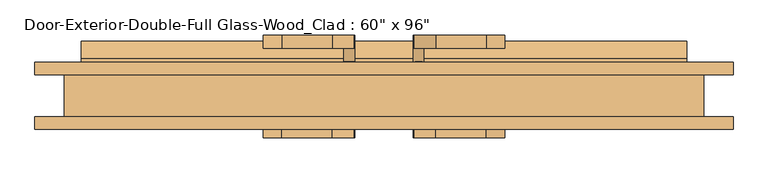
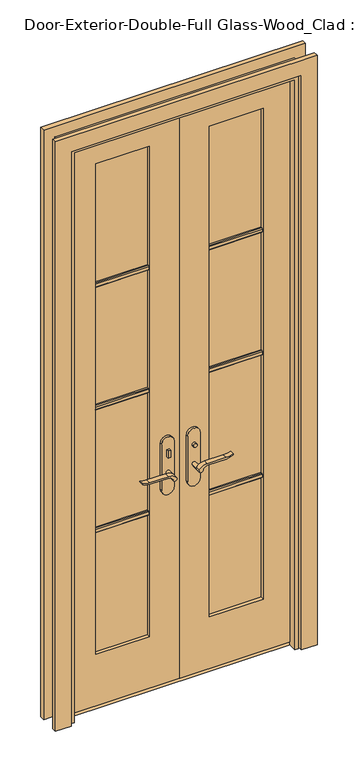
"""IFC4 building model written with IfcOpenShell, lengths in millimetres: door geometry."""

from ifc_helpers import new_model, si_unit, point, frame, frame_2d, origin, place, context, project, spatial, polyline, circle_curve, trimmed, segment, composite_curve, outline, extrude, faceted_brep, source, transform, mapped, element, save


def door_199e0ab3(model_context):
    return source(origin(), model_context, "Body", "SolidModel", [
        extrude(outline(polyline([(19.05, 12.7), (53.975, 12.7), (79.375, 0.0), (-6.35, 0.0), (19.05, 12.7)])), frame((-457.2, 0.0, 0.0), z_axis=(1.0, 0.0, 0.0), x_axis=(0.0, 1.0, 0.0)), (0.0, 0.0, 1.0), 914.4),
        extrude(outline(polyline([(-47.4019111, -26.35), (-57.4019111, -26.35), (-57.4019111, -16.35), (-47.4019111, -16.35), (-47.4019111, -26.35)])), frame((0.0, 0.0, 981.9), z_axis=(0.0, 0.0, 1.0), x_axis=(1.0, 0.0, 0.0)), (0.0, 0.0, 1.0), 30.0),
        extrude(outline(composite_curve([segment(trimmed(circle_curve(frame_2d((996.9, -52.4019111)), 8.0), [point((996.9, -60.4019111))], [point((996.9, -44.4019111))], False, "CARTESIAN"), True, "CONTINUOUS"), segment(trimmed(circle_curve(frame_2d((996.9, -52.4019111)), 8.0), [point((996.9, -44.4019111))], [point((996.9, -60.4019111))], False, "CARTESIAN"), True, "CONTINUOUS")], self_intersect=False)), frame((0.0, 38.575, 0.0), z_axis=(0.0, 1.0, 0.0), x_axis=(0.0, 0.0, 1.0)), (0.0, 0.0, 1.0), 10.0),
        extrude(outline(composite_curve([segment(trimmed(circle_curve(frame_2d((897.1555521, -76.0694241)), 37.2832219), [point((919.0523287, -45.8937749))], [point((934.4, -77.7693445))], False, "CARTESIAN"), True, "CONTINUOUS"), segment(polyline([(934.4, -77.7693445), (934.4, -154.045502)]), True, "CONTINUOUS"), segment(trimmed(circle_curve(frame_2d((1017.6850638, -153.9791202)), 83.2850902), [point((934.4, -154.045502))], [point((939.4, -182.4019111))], True, "CARTESIAN"), True, "CONTINUOUS"), segment(polyline([(939.4, -182.4019111), (936.6135558, -182.4019111)]), True, "CONTINUOUS"), segment(trimmed(circle_curve(frame_2d((986.6709207, -150.4622499)), 59.3791355), [point((936.6135558, -182.4019111))], [point((927.4, -154.045502))], False, "CARTESIAN"), True, "CONTINUOUS"), segment(polyline([(927.4, -154.045502), (927.4, -77.7881013)]), True, "CONTINUOUS"), segment(trimmed(circle_curve(frame_2d((909.2738613, -77.7881013)), 18.1261387), [point((927.4, -77.7881013))], [point((914.4, -60.4019111))], True, "CARTESIAN"), True, "CONTINUOUS"), segment(trimmed(circle_curve(frame_2d((914.4, -52.4019111)), 8.0), [point((914.4, -60.4019111))], [point((919.0523287, -45.8937749))], False, "CARTESIAN"), True, "CONTINUOUS")], self_intersect=False)), frame((0.0, -66.35, 0.0), z_axis=(0.0, 1.0, 0.0), x_axis=(0.0, 0.0, 1.0)), (0.0, 0.0, 1.0), 20.0),
        extrude(outline(composite_curve([segment(trimmed(circle_curve(frame_2d((914.4, -52.4019111)), 8.0), [point((914.3999903, -60.4019111))], [point((919.0523287, -45.8937749))], False, "CARTESIAN"), True, "CONTINUOUS"), segment(trimmed(circle_curve(frame_2d((897.1555521, -76.0694241)), 37.2832219), [point((919.0523287, -45.8937749))], [point((934.4, -77.7693445))], False, "CARTESIAN"), True, "CONTINUOUS"), segment(polyline([(934.4, -77.7693445), (934.4, -154.045502)]), True, "CONTINUOUS"), segment(trimmed(circle_curve(frame_2d((1017.6850638, -153.9791202)), 83.2850902), [point((934.4, -154.045502))], [point((939.4, -182.4019111))], True, "CARTESIAN"), True, "CONTINUOUS"), segment(polyline([(939.4, -182.4019111), (936.6135558, -182.4019111)]), True, "CONTINUOUS"), segment(trimmed(circle_curve(frame_2d((986.6709207, -150.4622499)), 59.3791355), [point((936.6135558, -182.4019111))], [point((927.4, -154.045502))], False, "CARTESIAN"), True, "CONTINUOUS"), segment(polyline([(927.4, -154.045502), (927.4, -77.788099)]), True, "CONTINUOUS"), segment(trimmed(circle_curve(frame_2d((909.2738682, -77.788099)), 18.1261318), [point((927.4, -77.788099))], [point((914.3999903, -60.4019111))], True, "CARTESIAN"), True, "CONTINUOUS")], self_intersect=False)), frame((0.0, 68.575, 0.0), z_axis=(0.0, 1.0, 0.0), x_axis=(0.0, 0.0, 1.0)), (0.0, 0.0, 1.0), 20.0),
        extrude(outline(composite_curve([segment(trimmed(circle_curve(frame_2d((914.4, -52.4019111)), 8.0), [point((914.4, -60.4019111))], [point((914.4, -44.4019111))], False, "CARTESIAN"), True, "CONTINUOUS"), segment(trimmed(circle_curve(frame_2d((914.4, -52.4019111)), 8.0), [point((914.4, -44.4019111))], [point((914.4, -60.4019111))], False, "CARTESIAN"), True, "CONTINUOUS")], self_intersect=False)), frame((0.0, -46.35, 0.0), z_axis=(0.0, 1.0, 0.0), x_axis=(0.0, 0.0, 1.0)), (0.0, 0.0, 1.0), 30.0),
        extrude(outline(composite_curve([segment(trimmed(circle_curve(frame_2d((914.4, -52.4019111)), 8.0), [point((914.4, -60.4019111))], [point((914.4, -44.4019111))], False, "CARTESIAN"), True, "CONTINUOUS"), segment(trimmed(circle_curve(frame_2d((914.4, -52.4019111)), 8.0), [point((914.4, -44.4019111))], [point((914.4, -60.4019111))], False, "CARTESIAN"), True, "CONTINUOUS")], self_intersect=False)), frame((0.0, 38.575, 0.0), z_axis=(0.0, 1.0, 0.0), x_axis=(0.0, 0.0, 1.0)), (0.0, 0.0, 1.0), 30.0),
        extrude(outline(composite_curve([segment(polyline([(844.4, -27.4019111), (1039.4, -27.4019111)]), True, "CONTINUOUS"), segment(trimmed(circle_curve(frame_2d((1039.4, -52.4019111)), 25.0), [point((1039.4, -27.4019111))], [point((1039.4, -77.4019111))], False, "CARTESIAN"), True, "CONTINUOUS"), segment(polyline([(1039.4, -77.4019111), (844.4, -77.4019111)]), True, "CONTINUOUS"), segment(trimmed(circle_curve(frame_2d((844.4, -52.4019111)), 25.0), [point((844.4, -77.4019111))], [point((844.4, -27.4019111))], False, "CARTESIAN"), True, "CONTINUOUS")], self_intersect=False)), frame((0.0, -16.35, 0.0), z_axis=(0.0, 1.0, 0.0), x_axis=(0.0, 0.0, 1.0)), (0.0, 0.0, 1.0), 10.0),
        extrude(outline(composite_curve([segment(polyline([(844.4, -27.4019111), (1039.4, -27.4019111)]), True, "CONTINUOUS"), segment(trimmed(circle_curve(frame_2d((1039.4, -52.4019111)), 25.0), [point((1039.4, -27.4019111))], [point((1039.4, -77.4019111))], False, "CARTESIAN"), True, "CONTINUOUS"), segment(polyline([(1039.4, -77.4019111), (844.4, -77.4019111)]), True, "CONTINUOUS"), segment(trimmed(circle_curve(frame_2d((844.4, -52.4019111)), 25.0), [point((844.4, -77.4019111))], [point((844.4, -27.4019111))], False, "CARTESIAN"), True, "CONTINUOUS")], self_intersect=False)), frame((0.0, 28.575, 0.0), z_axis=(0.0, 1.0, 0.0), x_axis=(0.0, 0.0, 1.0)), (0.0, 0.0, 1.0), 10.0),
        extrude(outline(polyline([(47.3875, 48.575), (57.3875, 48.575), (57.3875, 38.575), (47.3875, 38.575), (47.3875, 48.575)])), frame((0.0, 0.0, 981.9), z_axis=(0.0, 0.0, 1.0), x_axis=(1.0, 0.0, 0.0)), (0.0, 0.0, 1.0), 30.0),
        extrude(outline(composite_curve([segment(trimmed(circle_curve(frame_2d((996.9, 52.3875)), 8.0), [point((996.9, 60.3875))], [point((996.9, 44.3875))], False, "CARTESIAN"), True, "CONTINUOUS"), segment(trimmed(circle_curve(frame_2d((996.9, 52.3875)), 8.0), [point((996.9, 44.3875))], [point((996.9, 60.3875))], False, "CARTESIAN"), True, "CONTINUOUS")], self_intersect=False)), frame((0.0, -26.35, 0.0), z_axis=(0.0, 1.0, 0.0), x_axis=(0.0, 0.0, 1.0)), (0.0, 0.0, 1.0), 10.0),
        extrude(outline(composite_curve([segment(trimmed(circle_curve(frame_2d((914.4, 52.3875)), 8.0), [point((919.0523287, 45.8793637))], [point((914.4, 60.3875))], False, "CARTESIAN"), True, "CONTINUOUS"), segment(trimmed(circle_curve(frame_2d((909.2738613, 77.7736901)), 18.1261387), [point((914.4, 60.3875))], [point((927.4, 77.7736901))], True, "CARTESIAN"), True, "CONTINUOUS"), segment(polyline([(927.4, 77.7736901), (927.4, 154.0310909)]), True, "CONTINUOUS"), segment(trimmed(circle_curve(frame_2d((986.6709207, 150.4478388)), 59.3791355), [point((927.4, 154.0310909))], [point((936.6135558, 182.3875))], False, "CARTESIAN"), True, "CONTINUOUS"), segment(polyline([(936.6135558, 182.3875), (939.4, 182.3875)]), True, "CONTINUOUS"), segment(trimmed(circle_curve(frame_2d((1017.6850638, 153.9647091)), 83.2850902), [point((939.4, 182.3875))], [point((934.4, 154.0310909))], True, "CARTESIAN"), True, "CONTINUOUS"), segment(polyline([(934.4, 154.0310909), (934.4, 77.7549333)]), True, "CONTINUOUS"), segment(trimmed(circle_curve(frame_2d((897.1555521, 76.0550129)), 37.2832219), [point((934.4, 77.7549333))], [point((919.0523287, 45.8793637))], False, "CARTESIAN"), True, "CONTINUOUS")], self_intersect=False)), frame((0.0, 68.575, 0.0), z_axis=(0.0, 1.0, 0.0), x_axis=(0.0, 0.0, 1.0)), (0.0, 0.0, 1.0), 20.0),
        extrude(outline(composite_curve([segment(trimmed(circle_curve(frame_2d((909.2738682, 77.7736878)), 18.1261318), [point((914.3999903, 60.3875))], [point((927.4, 77.7736878))], True, "CARTESIAN"), True, "CONTINUOUS"), segment(polyline([(927.4, 77.7736878), (927.4, 154.0310909)]), True, "CONTINUOUS"), segment(trimmed(circle_curve(frame_2d((986.6709207, 150.4478388)), 59.3791355), [point((927.4, 154.0310909))], [point((936.6135558, 182.3875))], False, "CARTESIAN"), True, "CONTINUOUS"), segment(polyline([(936.6135558, 182.3875), (939.4, 182.3875)]), True, "CONTINUOUS"), segment(trimmed(circle_curve(frame_2d((1017.6850638, 153.9647091)), 83.2850902), [point((939.4, 182.3875))], [point((934.4, 154.0310909))], True, "CARTESIAN"), True, "CONTINUOUS"), segment(polyline([(934.4, 154.0310909), (934.4, 77.7549333)]), True, "CONTINUOUS"), segment(trimmed(circle_curve(frame_2d((897.1555521, 76.0550129)), 37.2832219), [point((934.4, 77.7549333))], [point((919.0523287, 45.8793637))], False, "CARTESIAN"), True, "CONTINUOUS"), segment(trimmed(circle_curve(frame_2d((914.4, 52.3875)), 8.0), [point((919.0523287, 45.8793637))], [point((914.3999903, 60.3875))], False, "CARTESIAN"), True, "CONTINUOUS")], self_intersect=False)), frame((0.0, -66.35, 0.0), z_axis=(0.0, 1.0, 0.0), x_axis=(0.0, 0.0, 1.0)), (0.0, 0.0, 1.0), 20.0),
        extrude(outline(composite_curve([segment(trimmed(circle_curve(frame_2d((914.4, 52.3875)), 8.0), [point((914.4, 60.3875))], [point((914.4, 44.3875))], False, "CARTESIAN"), True, "CONTINUOUS"), segment(trimmed(circle_curve(frame_2d((914.4, 52.3875)), 8.0), [point((914.4, 44.3875))], [point((914.4, 60.3875))], False, "CARTESIAN"), True, "CONTINUOUS")], self_intersect=False)), frame((0.0, 38.575, 0.0), z_axis=(0.0, 1.0, 0.0), x_axis=(0.0, 0.0, 1.0)), (0.0, 0.0, 1.0), 30.0),
        extrude(outline(composite_curve([segment(trimmed(circle_curve(frame_2d((914.4, 52.3875)), 8.0), [point((914.4, 60.3875))], [point((914.4, 44.3875))], False, "CARTESIAN"), True, "CONTINUOUS"), segment(trimmed(circle_curve(frame_2d((914.4, 52.3875)), 8.0), [point((914.4, 44.3875))], [point((914.4, 60.3875))], False, "CARTESIAN"), True, "CONTINUOUS")], self_intersect=False)), frame((0.0, -46.35, 0.0), z_axis=(0.0, 1.0, 0.0), x_axis=(0.0, 0.0, 1.0)), (0.0, 0.0, 1.0), 30.0),
        extrude(outline(composite_curve([segment(trimmed(circle_curve(frame_2d((844.4, 52.3875)), 25.0), [point((844.4, 27.3875))], [point((844.4, 77.3875))], False, "CARTESIAN"), True, "CONTINUOUS"), segment(polyline([(844.4, 77.3875), (1039.4, 77.3875)]), True, "CONTINUOUS"), segment(trimmed(circle_curve(frame_2d((1039.4, 52.3875)), 25.0), [point((1039.4, 77.3875))], [point((1039.4, 27.3875))], False, "CARTESIAN"), True, "CONTINUOUS"), segment(polyline([(1039.4, 27.3875), (844.4, 27.3875)]), True, "CONTINUOUS")], self_intersect=False)), frame((0.0, 28.575, 0.0), z_axis=(0.0, 1.0, 0.0), x_axis=(0.0, 0.0, 1.0)), (0.0, 0.0, 1.0), 10.0),
        extrude(outline(composite_curve([segment(trimmed(circle_curve(frame_2d((844.4, 52.3875)), 25.0), [point((844.4, 27.3875))], [point((844.4, 77.3875))], False, "CARTESIAN"), True, "CONTINUOUS"), segment(polyline([(844.4, 77.3875), (1039.4, 77.3875)]), True, "CONTINUOUS"), segment(trimmed(circle_curve(frame_2d((1039.4, 52.3875)), 25.0), [point((1039.4, 77.3875))], [point((1039.4, 27.3875))], False, "CARTESIAN"), True, "CONTINUOUS"), segment(polyline([(1039.4, 27.3875), (844.4, 27.3875)]), True, "CONTINUOUS")], self_intersect=False)), frame((0.0, -16.35, 0.0), z_axis=(0.0, 1.0, 0.0), x_axis=(0.0, 0.0, 1.0)), (0.0, 0.0, 1.0), 10.0),
        extrude(outline(polyline([(7.62, 1806.971875), (7.62, 1787.921875), (1.27, 1787.921875), (-1.905, 1791.096875), (-1.905, 1803.796875), (1.27, 1806.971875), (7.62, 1806.971875)])), frame((120.65, 0.0, 0.0), z_axis=(1.0, 0.0, 0.0), x_axis=(0.0, 1.0, 0.0)), (0.0, 0.0, 1.0), 215.9),
        extrude(outline(polyline([(7.62, 1285.08125), (7.62, 1266.03125), (1.27, 1266.03125), (-1.905, 1269.20625), (-1.905, 1281.90625), (1.27, 1285.08125), (7.62, 1285.08125)])), frame((120.65, 0.0, 0.0), z_axis=(1.0, 0.0, 0.0), x_axis=(0.0, 1.0, 0.0)), (0.0, 0.0, 1.0), 215.9),
        extrude(outline(polyline([(7.62, 763.190625), (7.62, 744.140625), (1.27, 744.140625), (-1.905, 747.315625), (-1.905, 760.015625), (1.27, 763.190625), (7.62, 763.190625)])), frame((120.65, 0.0, 0.0), z_axis=(1.0, 0.0, 0.0), x_axis=(0.0, 1.0, 0.0)), (0.0, 0.0, 1.0), 215.9),
        extrude(outline(polyline([(14.605, 1806.971875), (20.955, 1806.971875), (24.13, 1803.796875), (24.13, 1791.096875), (20.955, 1787.921875), (14.605, 1787.921875), (14.605, 1806.971875)])), frame((-336.55, 0.0, 0.0), z_axis=(1.0, 0.0, 0.0), x_axis=(0.0, 1.0, 0.0)), (0.0, 0.0, 1.0), 215.9),
        extrude(outline(polyline([(14.605, 1285.08125), (20.955, 1285.08125), (24.13, 1281.90625), (24.13, 1269.20625), (20.955, 1266.03125), (14.605, 1266.03125), (14.605, 1285.08125)])), frame((-336.55, 0.0, 0.0), z_axis=(1.0, 0.0, 0.0), x_axis=(0.0, 1.0, 0.0)), (0.0, 0.0, 1.0), 215.9),
        extrude(outline(polyline([(14.605, 763.190625), (20.955, 763.190625), (24.13, 760.015625), (24.13, 747.315625), (20.955, 744.140625), (14.605, 744.140625), (14.605, 763.190625)])), frame((-336.55, 0.0, 0.0), z_axis=(1.0, 0.0, 0.0), x_axis=(0.0, 1.0, 0.0)), (0.0, 0.0, 1.0), 215.9),
        extrude(outline(polyline([(14.605, 1806.971875), (20.955, 1806.971875), (24.13, 1803.796875), (24.13, 1791.096875), (20.955, 1787.921875), (14.605, 1787.921875), (14.605, 1806.971875)])), frame((120.65, 0.0, 0.0), z_axis=(1.0, 0.0, 0.0), x_axis=(0.0, 1.0, 0.0)), (0.0, 0.0, 1.0), 215.9),
        extrude(outline(polyline([(14.605, 1285.08125), (20.955, 1285.08125), (24.13, 1281.90625), (24.13, 1269.20625), (20.955, 1266.03125), (14.605, 1266.03125), (14.605, 1285.08125)])), frame((120.65, 0.0, 0.0), z_axis=(1.0, 0.0, 0.0), x_axis=(0.0, 1.0, 0.0)), (0.0, 0.0, 1.0), 215.9),
        extrude(outline(polyline([(14.605, 763.190625), (20.955, 763.190625), (24.13, 760.015625), (24.13, 747.315625), (20.955, 744.140625), (14.605, 744.140625), (14.605, 763.190625)])), frame((120.65, 0.0, 0.0), z_axis=(1.0, 0.0, 0.0), x_axis=(0.0, 1.0, 0.0)), (0.0, 0.0, 1.0), 215.9),
        extrude(outline(polyline([(7.62, 1806.971875), (7.62, 1787.921875), (1.27, 1787.921875), (-1.905, 1791.096875), (-1.905, 1803.796875), (1.27, 1806.971875), (7.62, 1806.971875)])), frame((-336.55, 0.0, 0.0), z_axis=(1.0, 0.0, 0.0), x_axis=(0.0, 1.0, 0.0)), (0.0, 0.0, 1.0), 215.9),
        extrude(outline(polyline([(7.62, 1285.08125), (7.62, 1266.03125), (1.27, 1266.03125), (-1.905, 1269.20625), (-1.905, 1281.90625), (1.27, 1285.08125), (7.62, 1285.08125)])), frame((-336.55, 0.0, 0.0), z_axis=(1.0, 0.0, 0.0), x_axis=(0.0, 1.0, 0.0)), (0.0, 0.0, 1.0), 215.9),
        extrude(outline(polyline([(7.62, 763.190625), (7.62, 744.140625), (1.27, 744.140625), (-1.905, 747.315625), (-1.905, 760.015625), (1.27, 763.190625), (7.62, 763.190625)])), frame((-336.55, 0.0, 0.0), z_axis=(1.0, 0.0, 0.0), x_axis=(0.0, 1.0, 0.0)), (0.0, 0.0, 1.0), 215.9),
        extrude(outline(polyline([(0.0, 463.55), (0.0, 527.05), (2508.25, 527.05), (2508.25, -527.05), (0.0, -527.05), (0.0, -463.55), (2444.75, -463.55), (2444.75, 463.55), (0.0, 463.55)])), frame((0.0, 28.575, 0.0), z_axis=(0.0, 1.0, 0.0), x_axis=(0.0, 0.0, 1.0)), (0.0, 0.0, 1.0), 19.05),
        extrude(outline(polyline([(0.0, 463.55), (0.0, 527.05), (2508.25, 527.05), (2508.25, -527.05), (0.0, -527.05), (0.0, -463.55), (2444.75, -463.55), (2444.75, 463.55), (0.0, 463.55)])), frame((0.0, -53.975, 0.0), z_axis=(0.0, 1.0, 0.0), x_axis=(0.0, 0.0, 1.0)), (0.0, 0.0, 1.0), 19.05),
        extrude(outline(polyline([(12.7, 457.2), (2438.4, 457.2), (2438.4, 1.5875), (12.7, 1.5875), (12.7, 457.2)]), holes=[polyline([(2319.3375, 120.65), (2319.3375, 336.55), (231.775, 336.55), (231.775, 120.65), (2319.3375, 120.65)])]), frame((0.0, -6.35, 0.0), z_axis=(0.0, 1.0, 0.0), x_axis=(0.0, 0.0, 1.0)), (0.0, 0.0, 1.0), 34.925),
        extrude(outline(polyline([(2438.4, -457.2), (12.7, -457.2), (12.7, -1.6019111), (2438.4, -1.6019111), (2438.4, -457.2)]), holes=[polyline([(231.775, -336.55), (2319.3375, -336.55), (2319.3375, -120.65), (231.775, -120.65), (231.775, -336.55)])]), frame((0.0, -6.35, 0.0), z_axis=(0.0, 1.0, 0.0), x_axis=(0.0, 0.0, 1.0)), (0.0, 0.0, 1.0), 34.925),
        faceted_brep([(482.6, 28.575, 0.0), (482.6, -34.925, 0.0), (457.2, -34.925, 0.0), (457.2, -41.275, 0.0), (444.5, -41.275, 0.0), (444.5, -6.35, 0.0), (457.2, -6.35, 0.0), (457.2, 28.575, 0.0), (482.6, 28.575, 2463.8), (482.6, -34.925, 2463.8), (-482.6, -34.925, 2463.8), (-482.6, -34.925, 0.0), (-457.2, -34.925, 0.0), (-457.2, -34.925, 2438.4), (457.2, -34.925, 2438.4), (457.2, -41.275, 2438.4), (-457.2, -41.275, 2438.4), (-457.2, -41.275, 0.0), (-444.5, -41.275, 0.0), (-444.5, -41.275, 2425.7), (444.5, -41.275, 2425.7), (444.5, -6.35, 2425.7), (1.5875, -6.35, 2425.7), (-1.6019111, -6.35, 2425.7), (-444.5, -6.35, 2425.7), (-444.5, -6.35, 0.0), (-457.2, -6.35, 0.0), (-457.2, -6.35, 2438.4), (-1.6019111, -6.35, 2438.4), (1.5875, -6.35, 2438.4), (457.2, -6.35, 2438.4), (457.2, 28.575, 2438.4), (1.5875, 28.575, 2438.4), (-1.6019111, 28.575, 2438.4), (-457.2, 28.575, 2438.4), (-457.2, 28.575, 0.0), (-482.6, 28.575, 0.0), (-482.6, 28.575, 2463.8)], [[[0, 1, 2, 3, 4, 5, 6, 7]], [[1, 0, 8, 9]], [[2, 1, 9, 10, 11, 12, 13, 14]], [[3, 2, 14, 15]], [[4, 3, 15, 16, 17, 18, 19, 20]], [[5, 4, 20, 21]], [[6, 5, 21, 22, 23, 24, 25, 26, 27, 28, 29, 30]], [[7, 6, 30, 31]], [[0, 7, 31, 32, 33, 34, 35, 36, 37, 8]], [[9, 8, 37, 10]], [[14, 13, 16, 15]], [[20, 19, 24, 23, 22, 21]], [[31, 30, 29, 28, 27, 34, 33, 32]], [[12, 11, 36, 35, 26, 25, 18, 17]], [[11, 10, 37, 36]], [[13, 12, 17, 16]], [[19, 18, 25, 24]], [[27, 26, 35, 34]]]),
        extrude(outline(polyline([(336.55, 7.62), (120.65, 7.62), (120.65, 14.605), (336.55, 14.605), (336.55, 7.62)])), frame((0.0, 0.0, 231.775), z_axis=(0.0, 0.0, 1.0), x_axis=(1.0, 0.0, 0.0)), (0.0, 0.0, 1.0), 2087.5625),
        extrude(outline(polyline([(-120.65, 7.62), (-336.55, 7.62), (-336.55, 14.605), (-120.65, 14.605), (-120.65, 7.62)])), frame((0.0, 0.0, 231.775), z_axis=(0.0, 0.0, 1.0), x_axis=(1.0, 0.0, 0.0)), (0.0, 0.0, 1.0), 2087.5625),
    ])


if __name__ == "__main__":
    model = new_model("IFC4")
    model_context = context("Model", 3, world=origin())
    ifc_project = project(units=[si_unit("LENGTHUNIT", "METRE", prefix="MILLI")], contexts=[model_context])
    site = spatial("IfcSite", under=ifc_project)
    building = spatial("IfcBuilding", under=site)
    placement = place(None, origin())
    door_shape = door_199e0ab3(model_context)
    element("IfcDoor", 1, ObjectType="Door-Exterior-Double-Full Glass-Wood_Clad : 60\" x 96\"", at=placement, inside=building, context=model_context, shape_type="MappedRepresentation", body=[
        mapped(door_shape, transform((0.0, 0.0, 0.0), x_axis=(1.0, 0.0, 0.0), y_axis=(0.0, 1.0, 0.0), z_axis=(0.0, 0.0, 1.0))),
    ])
    save(model, "model.ifc")

# Revit data of these elements
# Type "Door-Exterior-Double-Full Glass-Wood_Clad : 60\" x 96\""
#   Type Mark = "15"
#   Assembly Code = "B2030100"
#   Analytic Construction = "French door, wood frame with double glass"
#   Top Rail = 0' - 4 11/16"
#   Threshold Offset [instance default] = 0' - 0 1/2"
#   Thickness = 0' - 1 3/8"
#   Thermal Resistance (R) = 1.9158 (h·ft²·°F)/BTU
#   Swing Angle [instance default] = 90.00°
#   Stiles = 0' - 4 3/4"
#   Rough Width = 3' - 2"
#   Rough Height = 8' - 1"
#   Panel Width = 1' - 6"
#   Door Offset [instance default] = 0' - 0"
#   Height = 8' - 0"
#   Width = 3' - 0"
#   Heat Transfer Coefficient (U) = 0.5220 BTU/(h·ft²·°F)
#   Bottom Rail = 0' - 9 1/8"
#   Exterior Trim [instance default] = yes
#   Threshold [instance default] = yes
#   Show Grill [instance default] = yes
#   Function = 1
#   Trim Material = Cherry
#   Threshold Material = Cherry
#   Panel Material = Cherry
#   Glazing = Glass
#   Frame Material = Cherry
#   Door Handle Material = Aluminum
#   Visual Light Transmittance = 0
#   Solar Heat Gain Coefficient = 0
#   Wall Closure = (empty or 0)
#   Construction Type = (empty or 0)
# Element 1 (IfcDoor, "Door-Exterior-Double-Full Glass-Wood_Clad : 60\" x 96\"")
#   Materials on its faces: "Cherry", "Aluminum", "Glass"
# Materials
#   "Cherry": class "Wood", colour RGB 226 177 128, transparency 0, Description = "Prunus Serotina", Cost = 0
#   "Glass": class "Glass", colour RGB 0 128 192, transparency 0.75, Description = "Soda Lime Glass", Cost = 0
#   "Aluminum": class "Metal", colour RGB 247 247 247, transparency 0, Description = "Aluminum 6061", Cost = 0
